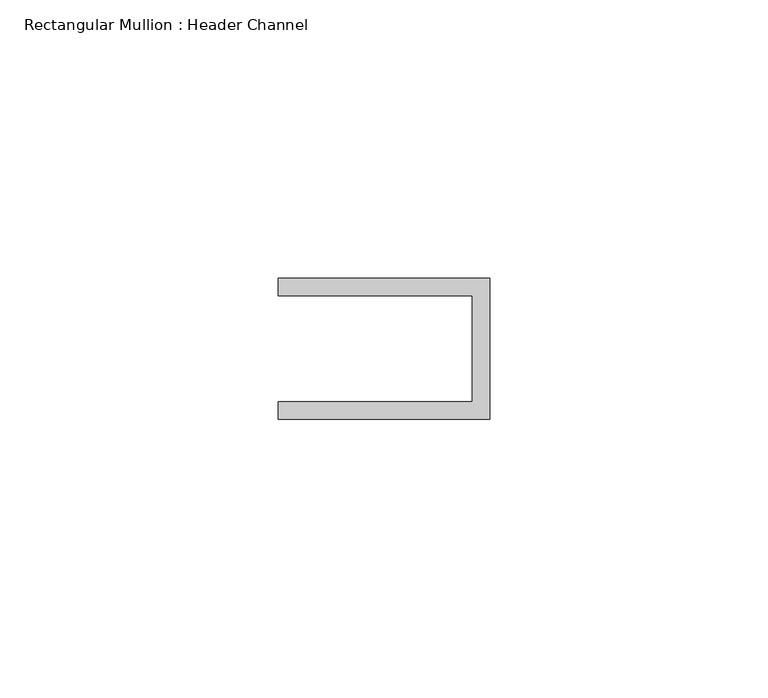
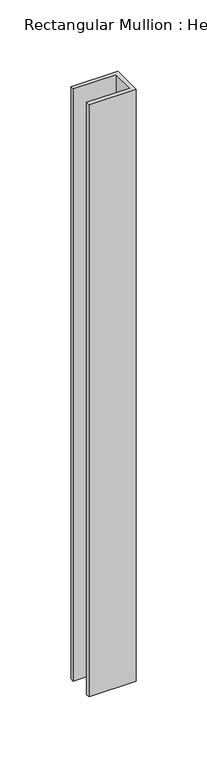
"""IFC4 building model written with IfcOpenShell, lengths in millimetres: member geometry, Rectangular Mullion : Header Channel."""

from ifc_helpers import new_model, si_unit, frame, origin, place, context, project, spatial, polyline, outline, extrude, source, transform, mapped, element, save


def rectangular_mullion_header_channel_2e58bf16(model_context):
    return source(origin(), model_context, "Body", "SweptSolid", [
        extrude(outline(polyline([(0.0, -12.7), (-38.1, -12.7), (-38.1, -9.525), (-3.175, -9.525), (-3.175, 9.525), (-38.1, 9.525), (-38.1, 12.7), (0.0, 12.7), (0.0, -12.7)])), frame((0.0, 0.0, -508.0), z_axis=(0.0, 0.0, 1.0), x_axis=(1.0, 0.0, 0.0)), (0.0, 0.0, 1.0), 508.0),
    ])


if __name__ == "__main__":
    model = new_model("IFC4")
    model_context = context("Model", 3, world=origin())
    ifc_project = project(units=[si_unit("LENGTHUNIT", "METRE", prefix="MILLI")], contexts=[model_context])
    site = spatial("IfcSite", under=ifc_project)
    building = spatial("IfcBuilding", under=site)
    placement = place(None, origin())
    rectangular_mullion_header_channel_shape = rectangular_mullion_header_channel_2e58bf16(model_context)
    element("IfcMember", 1, ObjectType="Rectangular Mullion : Header Channel", at=placement, inside=building, context=model_context, shape_type="MappedRepresentation", body=[
        mapped(rectangular_mullion_header_channel_shape, transform((0.0, 0.0, 0.0), x_axis=(1.0, 0.0, 0.0), y_axis=(0.0, 1.0, 0.0), z_axis=(0.0, 0.0, 1.0))),
    ])
    save(model, "model.ifc")

# Revit data of these elements
# Type "Rectangular Mullion : Header Channel"
#   built-in parameter 1007322 = 0.0833333 (stored number, unit not read)
#   built-in parameter 1007321 = -0.03125 (stored number, unit not read)
#   built-in parameter 1007320 = 0.0416667 (stored number, unit not read)
# Element 1 (IfcMember, "Rectangular Mullion : Header Channel")
#   Materials on its faces: "ALUM"
# Materials
#   "ALUM": class "Generic", colour RGB 157 157 157, transparency 0, Cost = 0
